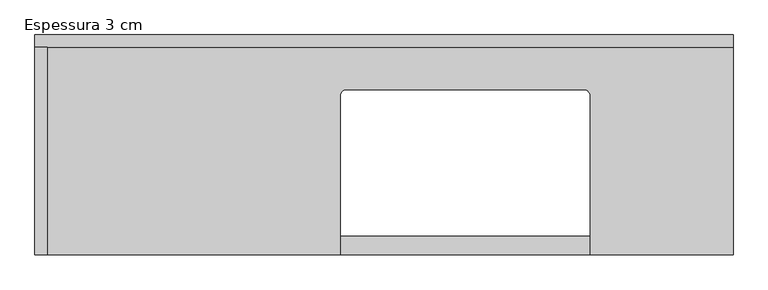
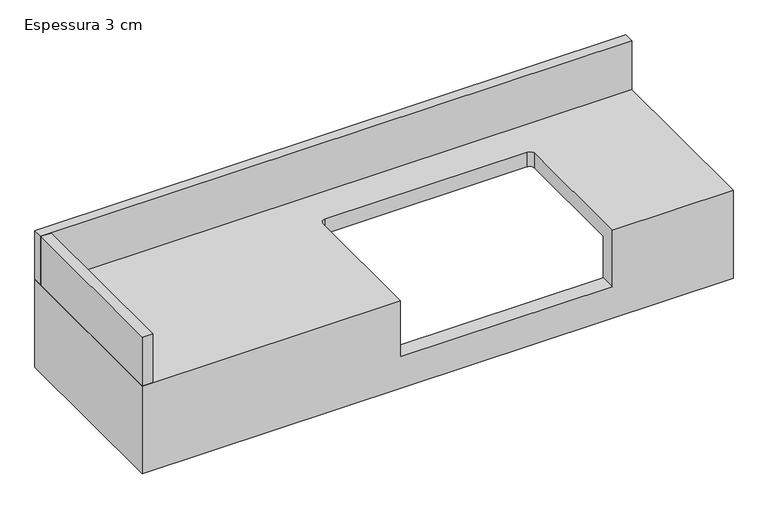
"""IFC4 building model written with IfcOpenShell, lengths in millimetres: furniture geometry, CC_BANCADA BANHEIRO COM CUBA_CANTO RETO : Espessura 3 cm."""

from ifc_helpers import new_model, si_unit, frame, origin, place, context, project, spatial, polyline, circle_curve, outline, extrude, source, transform, mapped, element, save
from ifc_brep_helpers import plane_surface, revolved_surface, advanced_brep


def espessura_3_cm_06997aab(model_context):
    return source(origin(), model_context, "Body", "SolidModel", [
        advanced_brep(
        [(750.0, 300.0, 860.0), (-394.0, 300.0, 860.0), (-394.0, -60.0, 860.0), (106.0, -60.0, 860.0), (106.0, 200.0, 860.0), (116.0, 210.0, 860.0), (506.0, 210.0, 860.0), (516.0, 200.0, 860.0), (516.0, -60.0, 860.0), (750.0, -60.0, 860.0), (750.0, 300.0, 680.0), (720.0, 300.0, 680.0), (720.0, 300.0, 830.0), (-364.0, 300.0, 830.0), (-364.0, 300.0, 680.0), (-394.0, 300.0, 680.0), (-394.0, -60.0, 680.0), (750.0, -60.0, 680.0), (516.0, -60.0, 745.0), (106.0, -60.0, 745.0), (720.0, -30.0, 830.0), (516.0, -30.0, 830.0), (516.0, 200.0, 830.0), (506.0, 210.0, 830.0), (116.0, 210.0, 830.0), (106.0, 200.0, 830.0), (106.0, -30.0, 830.0), (-364.0, -30.0, 830.0), (-364.0, -30.0, 680.0), (106.0, -30.0, 745.0), (516.0, -30.0, 745.0), (720.0, -30.0, 680.0)],
        [
            (0, 1),
            (1, 2),
            (2, 3),
            (3, 4),
            (4, 5, circle_curve(frame((116.0, 200.0, 860.0), z_axis=(0.0, 0.0, -1.0), x_axis=(0.0, 1.0, 0.0)), 10.0)),
            (5, 6),
            (6, 7, circle_curve(frame((506.0, 200.0, 860.0), z_axis=(0.0, 0.0, -1.0), x_axis=(0.0, 1.0, 0.0)), 10.0)),
            (7, 8),
            (8, 9),
            (9, 0),
            (0, 10),
            (10, 11),
            (11, 12),
            (12, 13),
            (13, 14),
            (14, 15),
            (15, 1),
            (15, 16),
            (16, 2),
            (16, 17),
            (17, 9),
            (8, 18),
            (18, 19),
            (19, 3),
            (17, 10),
            (12, 20),
            (20, 21),
            (21, 22),
            (22, 23, circle_curve(frame((506.0, 200.0, 830.0), z_axis=(0.0, 0.0, 1.0), x_axis=(0.0, 1.0, 0.0)), 10.0)),
            (23, 24),
            (24, 25, circle_curve(frame((116.0, 200.0, 830.0), z_axis=(0.0, 0.0, 1.0), x_axis=(0.0, 1.0, 0.0)), 10.0)),
            (25, 26),
            (26, 27),
            (27, 13),
            (27, 28),
            (28, 14),
            (26, 29),
            (29, 30),
            (30, 21),
            (20, 31),
            (31, 28),
            (11, 31),
            (5, 24),
            (23, 6),
            (18, 30),
            (29, 19),
            (4, 25),
            (7, 22),
        ],
        [
            plane_surface(frame((-394.0, 300.0, 860.0), z_axis=(0.0, 0.0, 1.0), x_axis=(-1.0, 0.0, 0.0))),
            plane_surface(frame((750.0, 300.0, 860.0), z_axis=(0.0, 1.0, 0.0), x_axis=(0.0, 0.0, -1.0))),
            plane_surface(frame((-394.0, 300.0, 860.0), z_axis=(-1.0, 0.0, 0.0), x_axis=(0.0, 0.0, -1.0))),
            plane_surface(frame((-394.0, -60.0, 860.0), z_axis=(0.0, -1.0, 0.0), x_axis=(0.0, 0.0, -1.0))),
            plane_surface(frame((750.0, -60.0, 860.0), z_axis=(1.0, 0.0, 0.0), x_axis=(0.0, 0.0, -1.0))),
            plane_surface(frame((-364.0, 300.0, 830.0), z_axis=(0.0, 0.0, -1.0), x_axis=(-1.0, 0.0, 0.0))),
            plane_surface(frame((-364.0, 300.0, 830.0), z_axis=(1.0, 0.0, 0.0), x_axis=(0.0, 0.0, -1.0))),
            plane_surface(frame((-364.0, -30.0, 830.0), z_axis=(0.0, 1.0, 0.0), x_axis=(0.0, 0.0, -1.0))),
            plane_surface(frame((720.0, -30.0, 830.0), z_axis=(-1.0, 0.0, 0.0), x_axis=(0.0, 0.0, -1.0))),
            plane_surface(frame((750.0, -60.0, 680.0), z_axis=(0.0, 0.0, -1.0), x_axis=(0.0, 1.0, 0.0))),
            plane_surface(frame((116.0, 210.0, 745.0), z_axis=(0.0, -1.0, 0.0), x_axis=(0.0, 0.0, 1.0))),
            plane_surface(frame((506.0, 210.0, 745.0), z_axis=(0.0, 0.0, 1.0), x_axis=(1.0, 0.0, 0.0))),
            revolved_surface(polyline([(116.0, 210.0, 830.0), (116.0, 210.0, 860.0)]), (116.0, 200.0, 900.0), (0.0, 0.0, -1.0)),
            plane_surface(frame((106.0, -190.0, 745.0), z_axis=(1.0, 0.0, 0.0), x_axis=(0.0, 0.0, 1.0))),
            plane_surface(frame((516.0, 200.0, 745.0), z_axis=(-1.0, 0.0, 0.0), x_axis=(0.0, 0.0, 1.0))),
            revolved_surface(polyline([(506.0, 210.0, 830.0), (506.0, 210.0, 860.0)]), (506.0, 200.0, 900.0), (0.0, 0.0, -1.0)),
        ],
        [
            (0, [[1, 2, 3, 4, 5, 6, 7, 8, 9, 10]]),
            (1, [[-1, 11, 12, 13, 14, 15, 16, 17]]),
            (2, [[-2, -17, 18, 19]]),
            (3, [[-3, -19, 20, 21, -9, 22, 23, 24]]),
            (4, [[-10, -21, 25, -11]]),
            (5, [[26, 27, 28, 29, 30, 31, 32, 33, 34, -14]]),
            (6, [[-34, 35, 36, -15]]),
            (7, [[-33, 37, 38, 39, -27, 40, 41, -35]]),
            (8, [[-26, -13, 42, -40]]),
            (9, [[-12, -25, -20, -18, -16, -36, -41, -42]]),
            (10, [[-6, 43, -30, 44]]),
            (11, [[-23, 45, -38, 46]]),
            (12, [[-5, 47, -31, -43]]),
            (13, [[-4, -24, -46, -37, -32, -47]]),
            (14, [[-8, 48, -28, -39, -45, -22]]),
            (15, [[-7, -44, -29, -48]]),
        ],
    ),
        extrude(outline(polyline([(-374.0, -60.0), (-394.0, -60.0), (-394.0, 280.0), (-374.0, 280.0), (-374.0, -60.0)])), frame((0.0, 0.0, 860.0), z_axis=(0.0, 0.0, 1.0), x_axis=(1.0, 0.0, 0.0)), (0.0, 0.0, 1.0), 100.0),
        extrude(outline(polyline([(750.0, 300.0), (750.0, 280.0), (-394.0, 280.0), (-394.0, 300.0), (750.0, 300.0)])), frame((0.0, 0.0, 860.0), z_axis=(0.0, 0.0, 1.0), x_axis=(1.0, 0.0, 0.0)), (0.0, 0.0, 1.0), 100.0),
    ])


if __name__ == "__main__":
    model = new_model("IFC4")
    model_context = context("Model", 3, world=origin())
    ifc_project = project(units=[si_unit("LENGTHUNIT", "METRE", prefix="MILLI")], contexts=[model_context])
    site = spatial("IfcSite", under=ifc_project)
    building = spatial("IfcBuilding", under=site)
    placement = place(None, origin())
    espessura_3_cm_shape = espessura_3_cm_06997aab(model_context)
    element("IfcFurniture", 1, ObjectType="CC_BANCADA BANHEIRO COM CUBA_CANTO RETO : Espessura 3 cm", at=placement, inside=building, context=model_context, shape_type="MappedRepresentation", body=[
        mapped(espessura_3_cm_shape, transform((0.0, 0.0, 0.0), x_axis=(1.0, 0.0, 0.0), y_axis=(0.0, 1.0, 0.0), z_axis=(0.0, 0.0, 1.0))),
    ])
    save(model, "model.ifc")

# Revit data of these elements
# Type "CC_BANCADA BANHEIRO COM CUBA_CANTO RETO : Espessura 3 cm"
#   Uso HS [instance default] = ""
#   h TESTEIRA AUX [instance default] = 0.15 m
#   Altura testeira [instance default] = 0.15 m
#   Altura rodapia [instance default] = 0.10 m
#   Espessura rodapia [instance default] = 0.02 m
#   Prof/2 [instance default] = 0.20 m
#   Offset cuba esquerda [instance default] = 0.40 m
#   Depth [instance default] = 1.20 m
#   Width [instance default] = 0.40 m
#   Espessura bancada = 0.03 m
#   Comprimento [instance default] = 1.20 m
#   Height [instance default] = 0.86 m
#   Testeira [instance default] = yes
#   Rodapia fundo [instance default] = no
#   Rodapia esquerda [instance default] = no
#   Rodapia direita [instance default] = no
#   Material porta-toalha [instance default] = .CROMADO
#   Material hidráulico [instance default] = .CROMADO
#   Material cuba [instance default] = .PORCELANA BRANCA
#   Material bancada [instance default] = .GRANITO_BRANCO_ITAUNAS
#   Assembly Code = ""
# Element 1 (IfcFurniture, "CC_BANCADA BANHEIRO COM CUBA_CANTO RETO : Espessura 3 cm")
#   Uso HS = "LAVABO"
#   Prof/2 = 0.18 m
#   Offset cuba esquerda = 0.50 m
#   Depth = 1.144 m
#   Width = 0.36 m
#   Comprimento = 1.144 m
#   Rodapia fundo = yes
#   Rodapia esquerda = yes
#   Materials on its faces: ".GRANITO_BRANCO_ITAUNAS"
# Materials
#   ".CROMADO": class "CC_METAIS", colour RGB 211 223 226, transparency 0, Cost = 0
#   ".PORCELANA BRANCA": class "CC_PORCELANA", colour RGB 230 230 230, transparency 0, Cost = 0
#   ".GRANITO_BRANCO_ITAUNAS": class ".CC_PEDRA REVEST.", colour RGB 202 195 174, transparency 0, Description = "Revestimento em granito", Cost = 0
